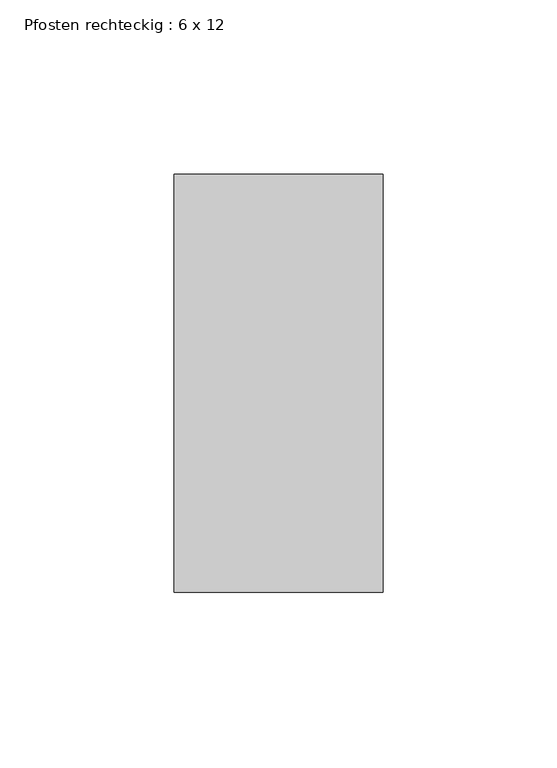
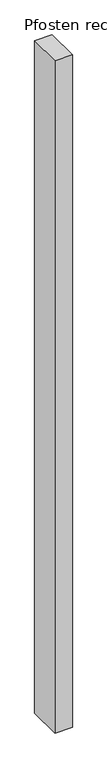
"""IFC4 building model written with IfcOpenShell, lengths in millimetres: member geometry, Pfosten rechteckig : 6 x 12."""

from ifc_helpers import new_model, si_unit, frame, origin, place, context, project, spatial, polyline, outline, extrude, source, transform, mapped, element, save


def pfosten_rechteckig_6_x_12_be5f7779(model_context):
    return source(origin(), model_context, "Body", "SweptSolid", [
        extrude(outline(polyline([(0.0, 60.0), (0.0, -60.0), (-60.0, -60.0), (-60.0, 60.0), (0.0, 60.0)])), frame((0.0, 0.0, -2440.0), z_axis=(0.0, 0.0, 1.0), x_axis=(1.0, 0.0, 0.0)), (0.0, 0.0, 1.0), 2440.0),
    ])


if __name__ == "__main__":
    model = new_model("IFC4")
    model_context = context("Model", 3, world=origin())
    ifc_project = project(units=[si_unit("LENGTHUNIT", "METRE", prefix="MILLI")], contexts=[model_context])
    site = spatial("IfcSite", under=ifc_project)
    building = spatial("IfcBuilding", under=site)
    placement = place(None, origin())
    pfosten_rechteckig_6_x_12_shape = pfosten_rechteckig_6_x_12_be5f7779(model_context)
    element("IfcMember", 1, ObjectType="Pfosten rechteckig : 6 x 12", at=placement, inside=building, context=model_context, shape_type="MappedRepresentation", body=[
        mapped(pfosten_rechteckig_6_x_12_shape, transform((0.0, 0.0, 0.0), x_axis=(1.0, 0.0, 0.0), y_axis=(0.0, 1.0, 0.0), z_axis=(0.0, 0.0, 1.0))),
    ])
    save(model, "model.ifc")

# Revit data of these elements
# Type "Pfosten rechteckig : 6 x 12"
#   built-in parameter 1007304 = 0.393701 (stored number, unit not read)
#   built-in parameter 1007301 = 0.0984252 (stored number, unit not read)
#   built-in parameter 1007300 = 0.0984252 (stored number, unit not read)
# Element 1 (IfcMember, "Pfosten rechteckig : 6 x 12")
#   Materials on its faces: "Metall - verzinkt"
# Materials
#   "Metall - verzinkt": class "Allgemeines", colour RGB 200 200 200, transparency 0, Cost = 0
